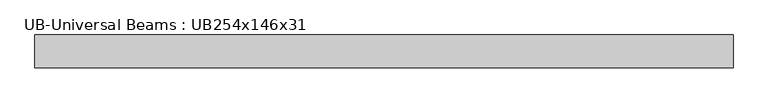
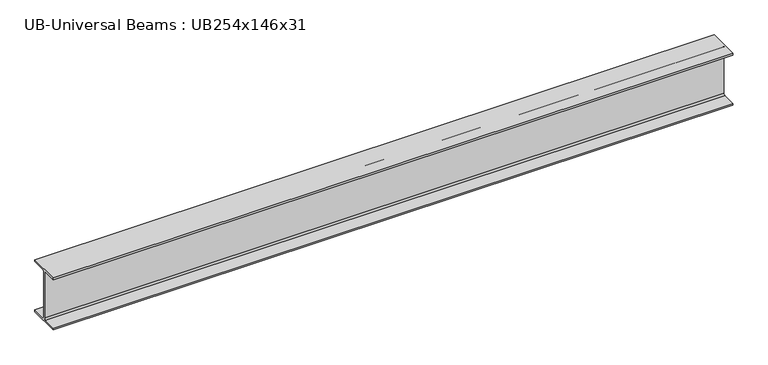
"""IFC4 building model written with IfcOpenShell, lengths in millimetres: beam geometry, UB-Universal Beams : UB254x146x31."""

from ifc_helpers import new_model, si_unit, point, frame, frame_2d, origin, place, context, project, spatial, polyline, circle_curve, trimmed, segment, composite_curve, outline, extrude, source, transform, mapped, element, save


def ub_universal_beams_ub254x146x31_beafa172(model_context):
    return source(origin(), model_context, "Body", "SweptSolid", [
        extrude(outline(composite_curve([segment(polyline([(73.05, -117.1), (73.05, -125.7), (-73.05, -125.7), (-73.05, -117.1), (-10.6, -117.1)]), True, "CONTINUOUS"), segment(trimmed(circle_curve(frame_2d((-10.6, -109.5)), 7.6), [point((-10.6, -117.1))], [point((-3.0, -109.5))], True, "CARTESIAN"), True, "CONTINUOUS"), segment(polyline([(-3.0, -109.5), (-3.0, 109.5)]), True, "CONTINUOUS"), segment(trimmed(circle_curve(frame_2d((-10.6, 109.5)), 7.6), [point((-3.0, 109.5))], [point((-10.6, 117.1))], True, "CARTESIAN"), True, "CONTINUOUS"), segment(polyline([(-10.6, 117.1), (-73.05, 117.1), (-73.05, 125.7), (73.05, 125.7), (73.05, 117.1), (10.6, 117.1)]), True, "CONTINUOUS"), segment(trimmed(circle_curve(frame_2d((10.6, 109.5)), 7.6), [point((10.6, 117.1))], [point((3.0, 109.5))], True, "CARTESIAN"), True, "CONTINUOUS"), segment(polyline([(3.0, 109.5), (3.0, -109.5)]), True, "CONTINUOUS"), segment(trimmed(circle_curve(frame_2d((10.6, -109.5)), 7.6), [point((3.0, -109.5))], [point((10.6, -117.1))], True, "CARTESIAN"), True, "CONTINUOUS"), segment(polyline([(10.6, -117.1), (73.05, -117.1)]), True, "CONTINUOUS")], self_intersect=False)), frame((-1552.9, 0.0, 0.0), z_axis=(1.0, 0.0, 0.0), x_axis=(0.0, 1.0, 0.0)), (0.0, 0.0, 1.0), 3105.8),
    ])


if __name__ == "__main__":
    model = new_model("IFC4")
    model_context = context("Model", 3, world=origin())
    ifc_project = project(units=[si_unit("LENGTHUNIT", "METRE", prefix="MILLI")], contexts=[model_context])
    site = spatial("IfcSite", under=ifc_project)
    building = spatial("IfcBuilding", under=site)
    placement = place(None, origin())
    ub_universal_beams_ub254x146x31_shape = ub_universal_beams_ub254x146x31_beafa172(model_context)
    element("IfcBeam", 1, ObjectType="UB-Universal Beams : UB254x146x31", at=placement, inside=building, context=model_context, shape_type="MappedRepresentation", body=[
        mapped(ub_universal_beams_ub254x146x31_shape, transform((0.0, 0.0, 0.0), x_axis=(1.0, 0.0, 0.0), y_axis=(0.0, 1.0, 0.0), z_axis=(0.0, 0.0, 1.0))),
    ])
    save(model, "model.ifc")

# Revit data of these elements
# Type "UB-Universal Beams : UB254x146x31"
#   Section Name Key = "UB254X146X31"
#   Width = 14.61 cm
#   Web Thickness = 0.6 cm
#   Web Fillet = 0.76 cm
#   Warping Constant = 66000.0 cm⁶
#   Torsional Moment of Inertia = 8.55 cm⁴
#   Section Area = 39.7 cm²
#   Plastic Modulus weak axis = 94.1 cm³
#   Plastic Modulus strong axis = 393.0 cm³
#   Nominal Weight = 31.10 kgf/m
#   Moment of Inertia weak axis = 448.00 cm⁴
#   Moment of Inertia strong axis = 4413.00 cm⁴
#   Height = 25.14 cm
#   Flange Thickness = 0.86 cm
#   Elastic Modulus weak axis = 61.3 cm³
#   Elastic Modulus strong axis = 351.0 cm³
#   Centroid Vertical = 12.57 cm
#   Centroid Horizontal = 7.305 cm
#   Bolt Spacing = 7.0 cm
#   Length [instance default] = 1500 mm
#   Structural Material [instance default] = Metal - Steel 43-275
#   Type Comments = ""
#   Assembly Code = ""
# Element 1 (IfcBeam, "UB-Universal Beams : UB254x146x31")
#   Materials on its faces: "Metal - Steel 43-275"
# Materials
#   "Metal - Steel 43-275": class "Metal", colour RGB 247 247 247, transparency 0, Cost = 0
